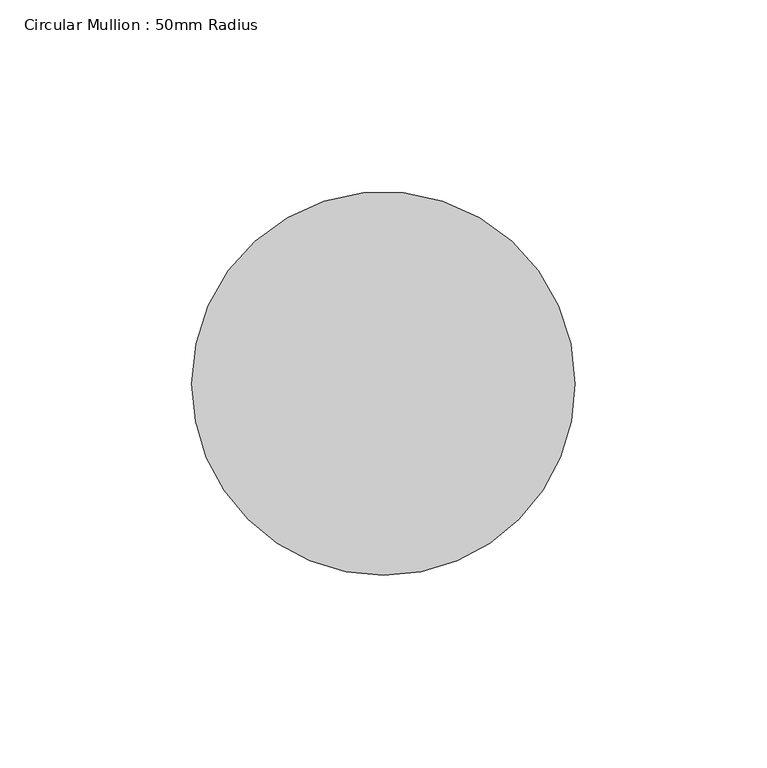
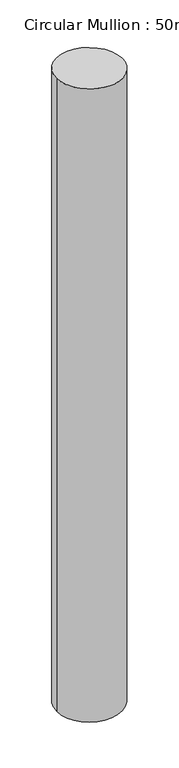
"""IFC4 building model written with IfcOpenShell, lengths in millimetres: member geometry, Circular Mullion : 50mm Radius."""

from ifc_helpers import new_model, si_unit, frame, origin, place, context, project, spatial, ellipse_curve, source, transform, mapped, element, save
from ifc_brep_helpers import plane_surface, cylinder_surface, advanced_brep


def circular_mullion_50mm_radius_eabd9903(model_context):
    return source(origin(), model_context, "Body", "AdvancedBrep", [
        advanced_brep(
        [(-100.0, 0.0, 2.2306316), (0.0, 0.0, 0.0), (0.0, 0.0, -1018.75699), (-100.0, 0.0, -1020.9430558)],
        [
            (0, 1, ellipse_curve(frame((-50.0, 0.0, 1.1153158), z_axis=(-0.022295368147964196, -0.02200703835660064, -0.9995091829602757), x_axis=(-0.7113444035948883, -0.7021451034481053, 0.03132719550298199)), 50.0245529, 50.0)),
            (1, 2),
            (2, 3, ellipse_curve(frame((-50.0, 0.0, -1019.8500229), z_axis=(-0.0218503523229633, -0.021567777597816744, 0.999528585420574), x_axis=(0.7113582122039032, 0.7021587334804863, 0.0307019042918533)), 50.0235818, 50.0)),
            (3, 0),
            (1, 0, ellipse_curve(frame((-50.0, 0.0, 1.1153158), z_axis=(-0.022295368147964196, -0.02200703835660064, -0.9995091829602757), x_axis=(-0.7113444035948883, -0.7021451034481053, 0.03132719550298199)), 50.0245529, 50.0)),
            (3, 2, ellipse_curve(frame((-50.0, 0.0, -1019.8500229), z_axis=(-0.0218503523229633, -0.021567777597816744, 0.999528585420574), x_axis=(0.7113582122039032, 0.7021587334804863, 0.0307019042918533)), 50.0235818, 50.0)),
        ],
        [
            cylinder_surface(frame((-50.0, 0.0, 0.0), z_axis=(0.0, 0.0, 1.0), x_axis=(1.0, 0.0, 0.0)), 50.0),
            plane_surface(frame((-214.1189207, 216.9242443, 0.0), z_axis=(0.0222953681479642, 0.022007038356600644, 0.9995091829602759), x_axis=(0.7113444035948878, 0.7021451034481059, -0.031327195502983476))),
            plane_surface(frame((-214.1189207, 216.9242443, -1018.75699), z_axis=(0.0218503523229633, 0.021567777597816744, -0.999528585420574), x_axis=(0.711358212203903, 0.7021587334804862, 0.030701904291859705))),
        ],
        [
            (0, [[1, 2, 3, 4]]),
            (0, [[5, -4, 6, -2]]),
            (1, [[-1, -5]]),
            (2, [[-6, -3]]),
        ],
    ),
    ])


if __name__ == "__main__":
    model = new_model("IFC4")
    model_context = context("Model", 3, world=origin())
    ifc_project = project(units=[si_unit("LENGTHUNIT", "METRE", prefix="MILLI")], contexts=[model_context])
    site = spatial("IfcSite", under=ifc_project)
    building = spatial("IfcBuilding", under=site)
    placement = place(None, origin())
    circular_mullion_50mm_radius_shape = circular_mullion_50mm_radius_eabd9903(model_context)
    element("IfcMember", 1, ObjectType="Circular Mullion : 50mm Radius", at=placement, inside=building, context=model_context, shape_type="MappedRepresentation", body=[
        mapped(circular_mullion_50mm_radius_shape, transform((0.0, 0.0, 0.0), x_axis=(1.0, 0.0, 0.0), y_axis=(0.0, 1.0, 0.0), z_axis=(0.0, 0.0, 1.0))),
    ])
    save(model, "model.ifc")

# Revit data of these elements
# Type "Circular Mullion : 50mm Radius"
#   built-in parameter 1007350 = 0.164042 (stored number, unit not read)
# Element 1 (IfcMember, "Circular Mullion : 50mm Radius")
#   Materials on its faces: "Aluminium"
# Materials
#   "Aluminium": class "Metal", colour RGB 247 247 247, transparency 0, Description = "Aluminium 6061", Cost = 0
